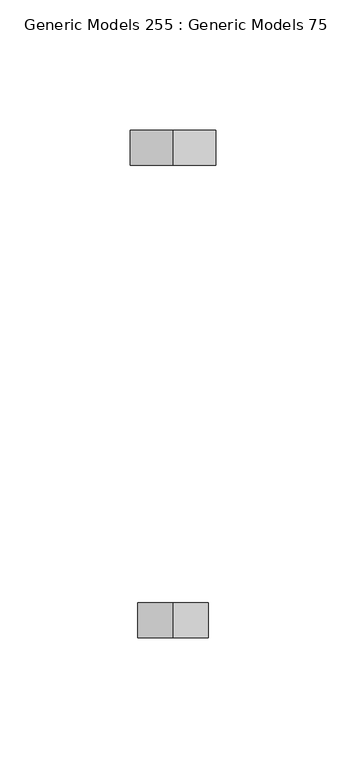
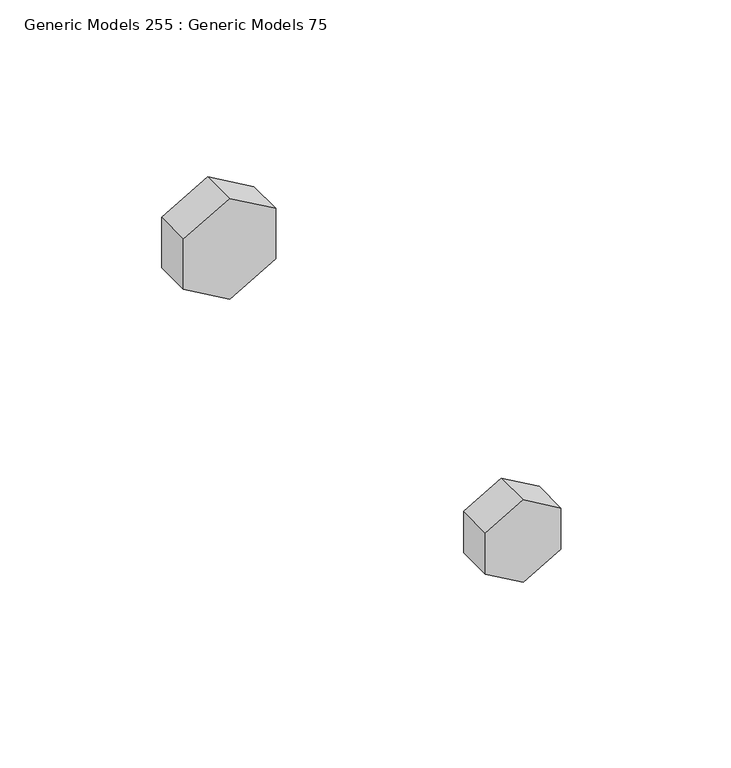
"""IFC4 building model written with IfcOpenShell, lengths in millimetres: proxy geometry, Generic Models 255 : Generic Models 75."""

from ifc_helpers import new_model, si_unit, frame, origin, place, context, project, spatial, polyline, outline, extrude, source, transform, mapped, element, save


def generic_models_255_generic_models_75_f19e14a3(model_context):
    return source(origin(), model_context, "Body", "SweptSolid", [
        extrude(outline(polyline([(266693.030998, 32006.2068618), (266712.080998, 32006.2068618), (266721.605998, 31989.7090778), (266712.080998, 31973.2112939), (266693.030998, 31973.2112939), (266683.505998, 31989.7090778), (266693.030998, 32006.2068618)])), frame((0.0, 35373.9582942, 0.0), z_axis=(0.0, 1.0, 0.0), x_axis=(0.0, 0.0, 1.0)), (0.0, 0.0, 1.0), 13.49375),
        extrude(outline(polyline([(266710.1638403, 31976.2187024), (266694.5864965, 31976.2187024), (266686.7978246, 31989.7090778), (266694.5864965, 32003.1994532), (266710.1638403, 32003.1994532), (266717.9525121, 31989.7090778), (266710.1638403, 31976.2187024)])), frame((0.0, 35192.1895442, 0.0), z_axis=(0.0, 1.0, 0.0), x_axis=(0.0, 0.0, 1.0)), (0.0, 0.0, 1.0), 13.49375),
    ])


if __name__ == "__main__":
    model = new_model("IFC4")
    model_context = context("Model", 3, world=origin())
    ifc_project = project(units=[si_unit("LENGTHUNIT", "METRE", prefix="MILLI")], contexts=[model_context])
    site = spatial("IfcSite", under=ifc_project)
    building = spatial("IfcBuilding", under=site)
    placement = place(None, origin())
    generic_models_255_generic_models_75_shape = generic_models_255_generic_models_75_f19e14a3(model_context)
    element("IfcBuildingElementProxy", 1, Name="Generic Models 255 : Generic Models 75", ObjectType="Generic Models 255 : Generic Models 75", at=placement, inside=building, context=model_context, shape_type="MappedRepresentation", body=[
        mapped(generic_models_255_generic_models_75_shape, transform((0.0, 0.0, 0.0), x_axis=(1.0, 0.0, 0.0), y_axis=(0.0, 1.0, 0.0), z_axis=(0.0, 0.0, 1.0))),
    ])
    save(model, "model.ifc")

# Revit data of these elements
# Element 1 (IfcBuildingElementProxy, "Generic Models 255 : Generic Models 75")
#   Materials on its faces: "3/4\" GALV. THRU BOLTS"
# Materials
#   "3/4\" GALV. THRU BOLTS": class "Generic", colour RGB 105 69 171, transparency 0, Cost = 0
